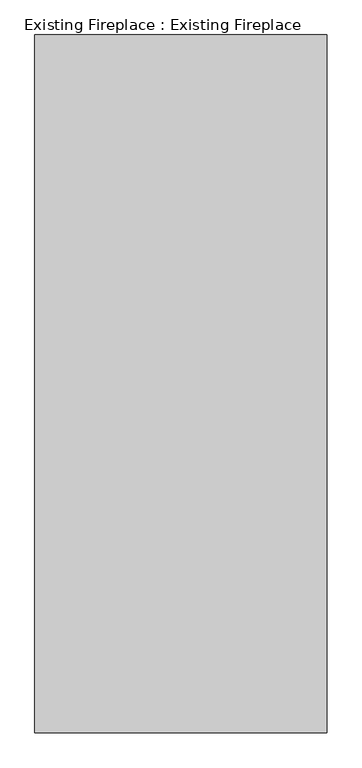
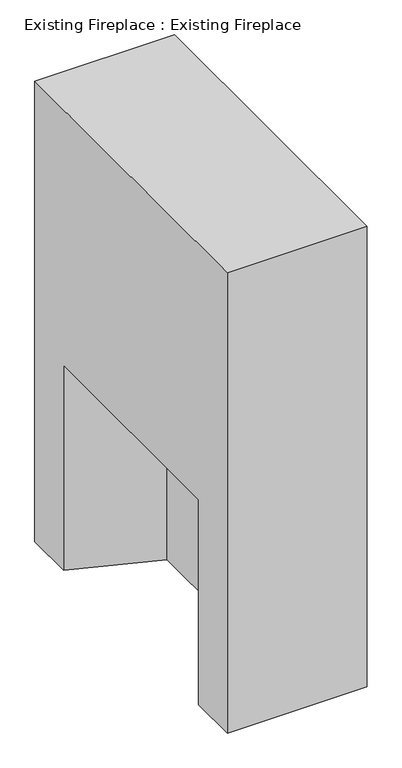
"""IFC4 building model written with IfcOpenShell, lengths in millimetres: proxy geometry, Existing Fireplace : Existing Fireplace."""

from ifc_helpers import new_model, si_unit, origin, place, context, project, spatial, faceted_brep, source, transform, mapped, element, save


def existing_fireplace_existing_fireplace_0dccdd15(model_context):
    return source(origin(), model_context, "Body", "Brep", [
        faceted_brep([(-1130.3962638, 2124.786172, 2743.2), (-1917.7962638, 2124.786172, 2743.2), (-1917.7962638, 245.186172, 2743.2), (-1130.3962638, 245.186172, 2743.2), (-1130.3962638, 2124.786172, 0.0), (-1130.3962638, 245.186172, 0.0), (-1511.3962638, 245.186172, 0.0), (-1816.1962638, 245.186172, 0.0), (-1917.7962638, 245.186172, 0.0), (-1917.7962638, 524.586172, 0.0), (-1435.1962638, 700.238207, 0.0), (-1435.1962638, 1669.7341369, 0.0), (-1917.7962638, 1845.386172, 0.0), (-1917.7962638, 2124.786172, 0.0), (-1816.1962638, 2124.786172, 0.0), (-1511.3962638, 2124.786172, 0.0), (-1917.7962638, 1845.386172, 1219.2), (-1917.7962638, 524.586172, 1219.2), (-1435.1962638, 1669.7341369, 1219.2), (-1435.1962638, 700.238207, 1219.2)], [[[0, 1, 2, 3]], [[4, 5, 6, 7, 8, 9, 10, 11, 12, 13, 14, 15]], [[1, 0, 4, 15, 14, 13]], [[2, 1, 13, 12, 16, 17, 9, 8]], [[3, 2, 8, 7, 6, 5]], [[0, 3, 5, 4]], [[16, 18, 19, 17]], [[17, 19, 10, 9]], [[19, 18, 11, 10]], [[18, 16, 12, 11]]]),
    ])


if __name__ == "__main__":
    model = new_model("IFC4")
    model_context = context("Model", 3, world=origin())
    ifc_project = project(units=[si_unit("LENGTHUNIT", "METRE", prefix="MILLI")], contexts=[model_context])
    site = spatial("IfcSite", under=ifc_project)
    building = spatial("IfcBuilding", under=site)
    placement = place(None, origin())
    existing_fireplace_existing_fireplace_shape = existing_fireplace_existing_fireplace_0dccdd15(model_context)
    element("IfcBuildingElementProxy", 1, Name="Existing Fireplace : Existing Fireplace", ObjectType="Existing Fireplace : Existing Fireplace", at=placement, inside=building, context=model_context, shape_type="MappedRepresentation", body=[
        mapped(existing_fireplace_existing_fireplace_shape, transform((0.0, 0.0, 0.0), x_axis=(1.0, 0.0, 0.0), y_axis=(0.0, 1.0, 0.0), z_axis=(0.0, 0.0, 1.0))),
    ])
    save(model, "model.ifc")

# Revit data of these elements
# Project information
#   Organization Name = "G3B Press"
#   Organization Description = "Paul F. Aubin Cosulting Services, Inc."
#   Building Name = "Revit Essentials for Architecture"
#   Author = "Paul F. Aubin"
#   Author Website = "https://www.paulaubin.com"
#   Copyright = "Copyright © 2020 Paul F Aubin, all rights reserved"
#   Project Issue Date = "8/1/2020"
#   Project Status = "Design Development"
#   Client Name = "Creating a Building Layout"
#   Project Address = "789 Main ST\nAnytown, IL 60000"
#   Project Name = "04 Residential_Complete"
#   Project Number = "2020.03A"
